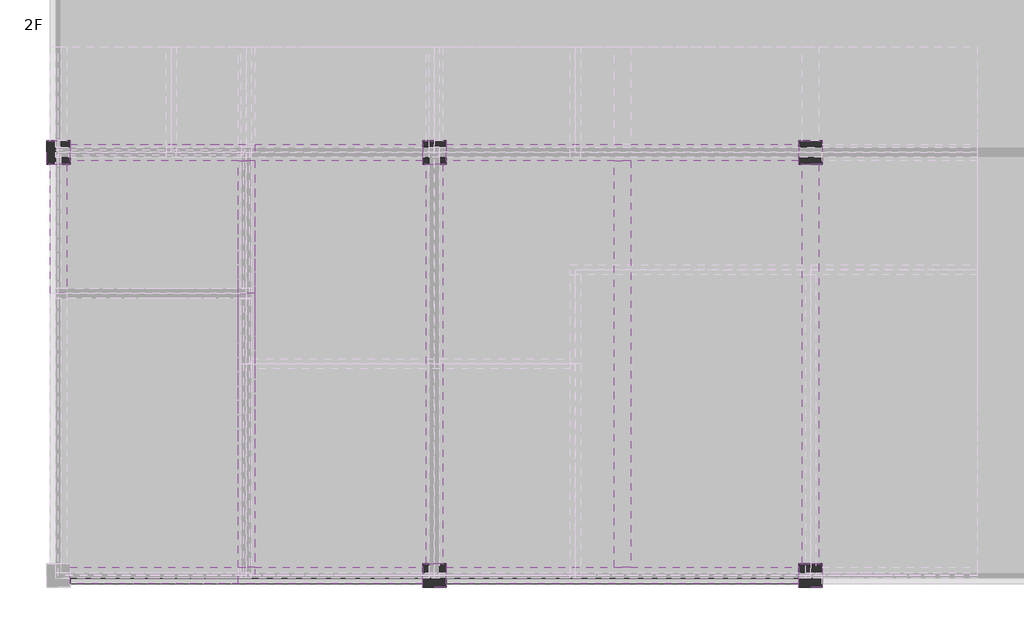
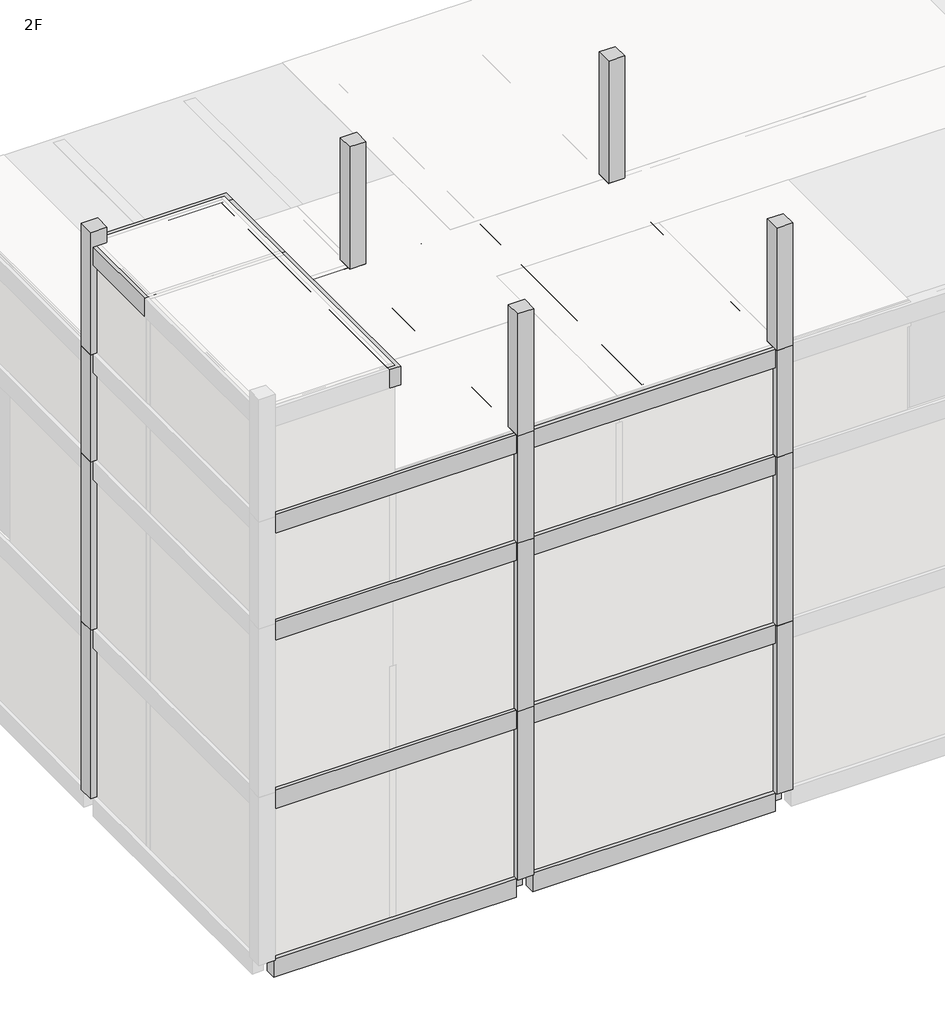
# One storey, part 4 of 7: 36 beams, 20 columns.
"""IFC4 building model written with IfcOpenShell, lengths in millimetres."""

from ifc_helpers import new_model, si_unit, frame, origin, place, context, project, spatial, polyline, outline, extrude, faceted_brep, element, save

model = new_model("IFC4")

# Units and contexts
model_context = context("Model", 3, world=origin())
ifc_project = project(units=[si_unit("LENGTHUNIT", "METRE", prefix="MILLI")], contexts=[model_context])

# Site, building, storey
site = spatial("IfcSite", under=ifc_project)
building = spatial("IfcBuilding", under=site)
storey = spatial("IfcBuildingStorey", under=building, Name="2F", Elevation=3500.0)

# Beams
placement = place(None, origin())
element("IfcBeam", 1, ObjectType="Concrete-Rectangular-Beam : BM111_400x500_RG1", at=placement, inside=storey, context=model_context, shape_type="Brep", body=[
    faceted_brep([(49634.6521483, 169923.8614395, 21500.0), (49284.6521483, 169923.8614395, 21500.0), (49284.6521483, 164098.8614395, 21500.0), (49284.6521483, 163748.8614395, 21500.0), (49634.6521483, 163748.8614395, 21500.0), (49634.6521483, 169923.8614395, 20900.0), (49634.6521483, 163748.8614395, 20900.0), (49284.6521483, 169923.8614395, 20900.0), (49284.6521483, 163748.8614395, 20900.0), (49284.6521483, 164098.8614395, 20900.0)], [[[0, 1, 2, 3, 4]], [[5, 0, 4, 6]], [[7, 5, 6, 8, 9]], [[1, 7, 9, 8, 3, 2]], [[4, 3, 8, 6]], [[1, 0, 5, 7]]]),
])
element("IfcBeam", 2, ObjectType="Concrete-Rectangular-Beam : BM111_400x500_RG1", at=placement, inside=storey, context=model_context, shape_type="Brep", body=[
    faceted_brep([(49634.6521483, 172748.8614395, 21500.0), (49634.6521483, 173098.8614395, 21500.0), (45709.6521483, 173098.8614395, 21500.0), (45709.6521483, 172748.8614395, 21500.0), (49284.6521483, 172748.8614395, 21500.0), (49634.6521483, 173098.8614395, 20900.0), (45709.6521483, 173098.8614395, 20900.0), (49634.6521483, 172748.8614395, 20900.0), (49284.6521483, 172748.8614395, 20900.0), (45709.6521483, 172748.8614395, 20900.0)], [[[0, 1, 2, 3, 4]], [[1, 5, 6, 2]], [[5, 7, 8, 9, 6]], [[7, 0, 4, 3, 9, 8]], [[1, 0, 7, 5]], [[3, 2, 6, 9]]]),
])
element("IfcBeam", 3, ObjectType="Concrete-Rectangular-Beam : BM111_400x500_RG1", at=placement, inside=storey, context=model_context, shape_type="SweptSolid", body=[
    extrude(outline(polyline([(49634.6521483, 169923.8614395), (49284.6521483, 169923.8614395), (49284.6521483, 172748.8614395), (49634.6521483, 172748.8614395), (49634.6521483, 169923.8614395)])), frame((0.0, 0.0, 20900.0), z_axis=(0.0, 0.0, 1.0), x_axis=(1.0, 0.0, 0.0)), (0.0, 0.0, 1.0), 600.0),
])
element("IfcBeam", 4, ObjectType="Concrete-Rectangular-Beam : BM111_400x500_RG1", at=placement, inside=storey, context=model_context, shape_type="SweptSolid", body=[
    extrude(outline(polyline([(45634.6521483, 169923.8614395), (45284.6521483, 169923.8614395), (45284.6521483, 172673.8614395), (45634.6521483, 172673.8614395), (45634.6521483, 169923.8614395)])), frame((0.0, 0.0, 20900.0), z_axis=(0.0, 0.0, 1.0), x_axis=(1.0, 0.0, 0.0)), (0.0, 0.0, 1.0), 600.0),
])
element("IfcBeam", 5, ObjectType="Concrete-Rectangular-Beam : BM111_400x500_RG1", at=placement, inside=storey, context=model_context, shape_type="SweptSolid", body=[
    extrude(outline(polyline([(49284.6521483, 172748.8614395), (49634.6521483, 172748.8614395), (49634.6521483, 164098.8614395), (49284.6521483, 164098.8614395), (49284.6521483, 172748.8614395)])), frame((0.0, 0.0, 2900.0), z_axis=(0.0, 0.0, 1.0), x_axis=(1.0, 0.0, 0.0)), (0.0, 0.0, 1.0), 600.0),
])
element("IfcBeam", 6, ObjectType="Concrete-Rectangular-Beam : BM111_400x500_RG1", at=placement, inside=storey, context=model_context, shape_type="SweptSolid", body=[
    extrude(outline(polyline([(57284.6521483, 172748.8614395), (57634.6521483, 172748.8614395), (57634.6521483, 164098.8614395), (57284.6521483, 164098.8614395), (57284.6521483, 172748.8614395)])), frame((0.0, 0.0, 2900.0), z_axis=(0.0, 0.0, 1.0), x_axis=(1.0, 0.0, 0.0)), (0.0, 0.0, 1.0), 600.0),
])
element("IfcBeam", 7, ObjectType="Concrete-Rectangular-Beam : BM111_400x500_RG1", at=placement, inside=storey, context=model_context, shape_type="SweptSolid", body=[
    extrude(outline(polyline([(49284.6521483, 172748.8614395), (49634.6521483, 172748.8614395), (49634.6521483, 164098.8614395), (49284.6521483, 164098.8614395), (49284.6521483, 172748.8614395)])), frame((0.0, 0.0, 8400.0), z_axis=(0.0, 0.0, 1.0), x_axis=(1.0, 0.0, 0.0)), (0.0, 0.0, 1.0), 600.0),
])
element("IfcBeam", 8, ObjectType="Concrete-Rectangular-Beam : BM111_400x500_RG1", at=placement, inside=storey, context=model_context, shape_type="SweptSolid", body=[
    extrude(outline(polyline([(57284.6521483, 172748.8614395), (57634.6521483, 172748.8614395), (57634.6521483, 164098.8614395), (57284.6521483, 164098.8614395), (57284.6521483, 172748.8614395)])), frame((0.0, 0.0, 8400.0), z_axis=(0.0, 0.0, 1.0), x_axis=(1.0, 0.0, 0.0)), (0.0, 0.0, 1.0), 600.0),
])
element("IfcBeam", 9, ObjectType="Concrete-Rectangular-Beam : BM111_400x500_RG1", at=placement, inside=storey, context=model_context, shape_type="SweptSolid", body=[
    extrude(outline(polyline([(49284.6521483, 172748.8614395), (49634.6521483, 172748.8614395), (49634.6521483, 164098.8614395), (49284.6521483, 164098.8614395), (49284.6521483, 172748.8614395)])), frame((0.0, 0.0, 13900.0), z_axis=(0.0, 0.0, 1.0), x_axis=(1.0, 0.0, 0.0)), (0.0, 0.0, 1.0), 600.0),
])
element("IfcBeam", 10, ObjectType="Concrete-Rectangular-Beam : BM111_400x500_RG1", at=placement, inside=storey, context=model_context, shape_type="SweptSolid", body=[
    extrude(outline(polyline([(57284.6521483, 172748.8614395), (57634.6521483, 172748.8614395), (57634.6521483, 164098.8614395), (57284.6521483, 164098.8614395), (57284.6521483, 172748.8614395)])), frame((0.0, 0.0, 13900.0), z_axis=(0.0, 0.0, 1.0), x_axis=(1.0, 0.0, 0.0)), (0.0, 0.0, 1.0), 600.0),
])
element("IfcBeam", 11, ObjectType="Concrete-Rectangular-Beam : BM111_400x500_RG1", at=placement, inside=storey, context=model_context, shape_type="SweptSolid", body=[
    extrude(outline(polyline([(49284.6521483, 172748.8614395), (49634.6521483, 172748.8614395), (49634.6521483, 164098.8614395), (49284.6521483, 164098.8614395), (49284.6521483, 172748.8614395)])), frame((0.0, 0.0, 17400.0), z_axis=(0.0, 0.0, 1.0), x_axis=(1.0, 0.0, 0.0)), (0.0, 0.0, 1.0), 600.0),
])
element("IfcBeam", 12, ObjectType="Concrete-Rectangular-Beam : BM111_400x500_RG1", at=placement, inside=storey, context=model_context, shape_type="SweptSolid", body=[
    extrude(outline(polyline([(57284.6521483, 172748.8614395), (57634.6521483, 172748.8614395), (57634.6521483, 164098.8614395), (57284.6521483, 164098.8614395), (57284.6521483, 172748.8614395)])), frame((0.0, 0.0, 17400.0), z_axis=(0.0, 0.0, 1.0), x_axis=(1.0, 0.0, 0.0)), (0.0, 0.0, 1.0), 600.0),
])
element("IfcBeam", 13, ObjectType="Concrete-Rectangular-Beam : BM111_400x500_RG1", at=placement, inside=storey, context=model_context, shape_type="Brep", body=[
    faceted_brep([(45709.6521483, 173098.8614395, 3500.0), (45709.6521483, 172748.8614395, 3500.0), (49284.6521483, 172748.8614395, 3500.0), (49634.6521483, 172748.8614395, 3500.0), (53209.6521483, 172748.8614395, 3500.0), (53209.6521483, 173098.8614395, 3500.0), (49634.6521483, 173098.8614395, 3500.0), (49284.6521483, 173098.8614395, 3500.0), (45709.6521483, 172748.8614395, 2900.0), (49284.6521483, 172748.8614395, 2900.0), (49634.6521483, 172748.8614395, 2900.0), (53209.6521483, 172748.8614395, 2900.0), (45709.6521483, 173098.8614395, 2900.0), (49284.6521483, 173098.8614395, 2900.0), (49634.6521483, 173098.8614395, 2900.0), (53209.6521483, 173098.8614395, 2900.0)], [[[0, 1, 2, 3, 4, 5, 6, 7]], [[1, 8, 9, 10, 11, 4, 3, 2]], [[8, 12, 13, 14, 15, 11, 10, 9]], [[12, 0, 7, 6, 5, 15, 14, 13]], [[1, 0, 12, 8]], [[5, 4, 11, 15]]]),
])
element("IfcBeam", 14, ObjectType="Concrete-Rectangular-Beam : BM111_400x500_RG1", at=placement, inside=storey, context=model_context, shape_type="Brep", body=[
    faceted_brep([(53709.6521483, 173098.8614395, 3500.0), (53709.6521483, 172748.8614395, 3500.0), (57284.6521483, 172748.8614395, 3500.0), (57634.6521483, 172748.8614395, 3500.0), (61209.6521483, 172748.8614395, 3500.0), (61209.6521483, 173098.8614395, 3500.0), (57634.6521483, 173098.8614395, 3500.0), (57284.6521483, 173098.8614395, 3500.0), (53709.6521483, 172748.8614395, 2900.0), (57284.6521483, 172748.8614395, 2900.0), (57634.6521483, 172748.8614395, 2900.0), (61209.6521483, 172748.8614395, 2900.0), (53709.6521483, 173098.8614395, 2900.0), (57284.6521483, 173098.8614395, 2900.0), (57634.6521483, 173098.8614395, 2900.0), (61209.6521483, 173098.8614395, 2900.0)], [[[0, 1, 2, 3, 4, 5, 6, 7]], [[1, 8, 9, 10, 11, 4, 3, 2]], [[8, 12, 13, 14, 15, 11, 10, 9]], [[12, 0, 7, 6, 5, 15, 14, 13]], [[1, 0, 12, 8]], [[5, 4, 11, 15]]]),
])
element("IfcBeam", 15, ObjectType="Concrete-Rectangular-Beam : BM111_400x500_RG1", at=placement, inside=storey, context=model_context, shape_type="Brep", body=[
    faceted_brep([(45709.6521483, 164098.8614395, 3500.0), (45709.6521483, 163748.8614395, 3500.0), (53209.6521483, 163748.8614395, 3500.0), (53209.6521483, 164098.8614395, 3500.0), (49634.6521483, 164098.8614395, 3500.0), (49284.6521483, 164098.8614395, 3500.0), (45709.6521483, 163748.8614395, 2900.0), (53209.6521483, 163748.8614395, 2900.0), (45709.6521483, 164098.8614395, 2900.0), (49284.6521483, 164098.8614395, 2900.0), (49634.6521483, 164098.8614395, 2900.0), (53209.6521483, 164098.8614395, 2900.0)], [[[0, 1, 2, 3, 4, 5]], [[1, 6, 7, 2]], [[6, 8, 9, 10, 11, 7]], [[8, 0, 5, 4, 3, 11, 10, 9]], [[1, 0, 8, 6]], [[3, 2, 7, 11]]]),
])
element("IfcBeam", 16, ObjectType="Concrete-Rectangular-Beam : BM111_400x500_RG1", at=placement, inside=storey, context=model_context, shape_type="Brep", body=[
    faceted_brep([(53709.6521483, 164098.8614395, 3500.0), (53709.6521483, 163748.8614395, 3500.0), (61209.6521483, 163748.8614395, 3500.0), (61209.6521483, 164098.8614395, 3500.0), (57634.6521483, 164098.8614395, 3500.0), (57284.6521483, 164098.8614395, 3500.0), (53709.6521483, 163748.8614395, 2900.0), (61209.6521483, 163748.8614395, 2900.0), (53709.6521483, 164098.8614395, 2900.0), (57284.6521483, 164098.8614395, 2900.0), (57634.6521483, 164098.8614395, 2900.0), (61209.6521483, 164098.8614395, 2900.0)], [[[0, 1, 2, 3, 4, 5]], [[1, 6, 7, 2]], [[6, 8, 9, 10, 11, 7]], [[8, 0, 5, 4, 3, 11, 10, 9]], [[1, 0, 8, 6]], [[3, 2, 7, 11]]]),
])
element("IfcBeam", 17, ObjectType="Concrete-Rectangular-Beam : BM111_400x500_RG1", at=placement, inside=storey, context=model_context, shape_type="Brep", body=[
    faceted_brep([(45709.6521483, 173098.8614395, 9000.0), (45709.6521483, 172748.8614395, 9000.0), (49284.6521483, 172748.8614395, 9000.0), (49634.6521483, 172748.8614395, 9000.0), (53209.6521483, 172748.8614395, 9000.0), (53209.6521483, 173098.8614395, 9000.0), (49634.6521483, 173098.8614395, 9000.0), (49284.6521483, 173098.8614395, 9000.0), (45709.6521483, 172748.8614395, 8400.0), (49284.6521483, 172748.8614395, 8400.0), (49634.6521483, 172748.8614395, 8400.0), (53209.6521483, 172748.8614395, 8400.0), (45709.6521483, 173098.8614395, 8400.0), (49284.6521483, 173098.8614395, 8400.0), (49634.6521483, 173098.8614395, 8400.0), (53209.6521483, 173098.8614395, 8400.0)], [[[0, 1, 2, 3, 4, 5, 6, 7]], [[1, 8, 9, 10, 11, 4, 3, 2]], [[8, 12, 13, 14, 15, 11, 10, 9]], [[12, 0, 7, 6, 5, 15, 14, 13]], [[1, 0, 12, 8]], [[5, 4, 11, 15]]]),
])
element("IfcBeam", 18, ObjectType="Concrete-Rectangular-Beam : BM111_400x500_RG1", at=placement, inside=storey, context=model_context, shape_type="Brep", body=[
    faceted_brep([(53709.6521483, 173098.8614395, 9000.0), (53709.6521483, 172748.8614395, 9000.0), (57284.6521483, 172748.8614395, 9000.0), (57634.6521483, 172748.8614395, 9000.0), (61209.6521483, 172748.8614395, 9000.0), (61209.6521483, 173098.8614395, 9000.0), (57634.6521483, 173098.8614395, 9000.0), (57284.6521483, 173098.8614395, 9000.0), (53709.6521483, 172748.8614395, 8400.0), (57284.6521483, 172748.8614395, 8400.0), (57634.6521483, 172748.8614395, 8400.0), (61209.6521483, 172748.8614395, 8400.0), (53709.6521483, 173098.8614395, 8400.0), (57284.6521483, 173098.8614395, 8400.0), (57634.6521483, 173098.8614395, 8400.0), (61209.6521483, 173098.8614395, 8400.0)], [[[0, 1, 2, 3, 4, 5, 6, 7]], [[1, 8, 9, 10, 11, 4, 3, 2]], [[8, 12, 13, 14, 15, 11, 10, 9]], [[12, 0, 7, 6, 5, 15, 14, 13]], [[1, 0, 12, 8]], [[5, 4, 11, 15]]]),
])
element("IfcBeam", 19, ObjectType="Concrete-Rectangular-Beam : BM111_400x500_RG1", at=placement, inside=storey, context=model_context, shape_type="Brep", body=[
    faceted_brep([(45709.6521483, 164098.8614395, 9000.0), (45709.6521483, 163748.8614395, 9000.0), (53209.6521483, 163748.8614395, 9000.0), (53209.6521483, 164098.8614395, 9000.0), (49634.6521483, 164098.8614395, 9000.0), (49284.6521483, 164098.8614395, 9000.0), (45709.6521483, 163748.8614395, 8400.0), (53209.6521483, 163748.8614395, 8400.0), (45709.6521483, 164098.8614395, 8400.0), (49284.6521483, 164098.8614395, 8400.0), (49634.6521483, 164098.8614395, 8400.0), (53209.6521483, 164098.8614395, 8400.0)], [[[0, 1, 2, 3, 4, 5]], [[1, 6, 7, 2]], [[6, 8, 9, 10, 11, 7]], [[8, 0, 5, 4, 3, 11, 10, 9]], [[1, 0, 8, 6]], [[3, 2, 7, 11]]]),
])
element("IfcBeam", 20, ObjectType="Concrete-Rectangular-Beam : BM111_400x500_RG1", at=placement, inside=storey, context=model_context, shape_type="Brep", body=[
    faceted_brep([(53709.6521483, 164098.8614395, 9000.0), (53709.6521483, 163748.8614395, 9000.0), (61209.6521483, 163748.8614395, 9000.0), (61209.6521483, 164098.8614395, 9000.0), (57634.6521483, 164098.8614395, 9000.0), (57284.6521483, 164098.8614395, 9000.0), (53709.6521483, 163748.8614395, 8400.0), (61209.6521483, 163748.8614395, 8400.0), (53709.6521483, 164098.8614395, 8400.0), (57284.6521483, 164098.8614395, 8400.0), (57634.6521483, 164098.8614395, 8400.0), (61209.6521483, 164098.8614395, 8400.0)], [[[0, 1, 2, 3, 4, 5]], [[1, 6, 7, 2]], [[6, 8, 9, 10, 11, 7]], [[8, 0, 5, 4, 3, 11, 10, 9]], [[1, 0, 8, 6]], [[3, 2, 7, 11]]]),
])
element("IfcBeam", 21, ObjectType="Concrete-Rectangular-Beam : BM111_400x500_RG1", at=placement, inside=storey, context=model_context, shape_type="Brep", body=[
    faceted_brep([(45709.6521483, 173098.8614395, 14500.0), (45709.6521483, 172748.8614395, 14500.0), (49284.6521483, 172748.8614395, 14500.0), (49634.6521483, 172748.8614395, 14500.0), (53209.6521483, 172748.8614395, 14500.0), (53209.6521483, 173098.8614395, 14500.0), (49634.6521483, 173098.8614395, 14500.0), (49284.6521483, 173098.8614395, 14500.0), (45709.6521483, 172748.8614395, 13900.0), (49284.6521483, 172748.8614395, 13900.0), (49634.6521483, 172748.8614395, 13900.0), (53209.6521483, 172748.8614395, 13900.0), (45709.6521483, 173098.8614395, 13900.0), (49284.6521483, 173098.8614395, 13900.0), (49634.6521483, 173098.8614395, 13900.0), (53209.6521483, 173098.8614395, 13900.0)], [[[0, 1, 2, 3, 4, 5, 6, 7]], [[1, 8, 9, 10, 11, 4, 3, 2]], [[8, 12, 13, 14, 15, 11, 10, 9]], [[12, 0, 7, 6, 5, 15, 14, 13]], [[1, 0, 12, 8]], [[5, 4, 11, 15]]]),
])
element("IfcBeam", 22, ObjectType="Concrete-Rectangular-Beam : BM111_400x500_RG1", at=placement, inside=storey, context=model_context, shape_type="Brep", body=[
    faceted_brep([(53709.6521483, 173098.8614395, 14500.0), (53709.6521483, 172748.8614395, 14500.0), (57284.6521483, 172748.8614395, 14500.0), (57634.6521483, 172748.8614395, 14500.0), (61209.6521483, 172748.8614395, 14500.0), (61209.6521483, 173098.8614395, 14500.0), (57634.6521483, 173098.8614395, 14500.0), (57284.6521483, 173098.8614395, 14500.0), (53709.6521483, 172748.8614395, 13900.0), (57284.6521483, 172748.8614395, 13900.0), (57634.6521483, 172748.8614395, 13900.0), (61209.6521483, 172748.8614395, 13900.0), (53709.6521483, 173098.8614395, 13900.0), (57284.6521483, 173098.8614395, 13900.0), (57634.6521483, 173098.8614395, 13900.0), (61209.6521483, 173098.8614395, 13900.0)], [[[0, 1, 2, 3, 4, 5, 6, 7]], [[1, 8, 9, 10, 11, 4, 3, 2]], [[8, 12, 13, 14, 15, 11, 10, 9]], [[12, 0, 7, 6, 5, 15, 14, 13]], [[1, 0, 12, 8]], [[5, 4, 11, 15]]]),
])
element("IfcBeam", 23, ObjectType="Concrete-Rectangular-Beam : BM111_400x500_RG1", at=placement, inside=storey, context=model_context, shape_type="Brep", body=[
    faceted_brep([(45709.6521483, 164098.8614395, 14500.0), (45709.6521483, 163748.8614395, 14500.0), (53209.6521483, 163748.8614395, 14500.0), (53209.6521483, 164098.8614395, 14500.0), (49634.6521483, 164098.8614395, 14500.0), (49284.6521483, 164098.8614395, 14500.0), (45709.6521483, 163748.8614395, 13900.0), (53209.6521483, 163748.8614395, 13900.0), (45709.6521483, 164098.8614395, 13900.0), (49284.6521483, 164098.8614395, 13900.0), (49634.6521483, 164098.8614395, 13900.0), (53209.6521483, 164098.8614395, 13900.0)], [[[0, 1, 2, 3, 4, 5]], [[1, 6, 7, 2]], [[6, 8, 9, 10, 11, 7]], [[8, 0, 5, 4, 3, 11, 10, 9]], [[1, 0, 8, 6]], [[3, 2, 7, 11]]]),
])
element("IfcBeam", 24, ObjectType="Concrete-Rectangular-Beam : BM111_400x500_RG1", at=placement, inside=storey, context=model_context, shape_type="Brep", body=[
    faceted_brep([(53709.6521483, 164098.8614395, 14500.0), (53709.6521483, 163748.8614395, 14500.0), (61209.6521483, 163748.8614395, 14500.0), (61209.6521483, 164098.8614395, 14500.0), (57634.6521483, 164098.8614395, 14500.0), (57284.6521483, 164098.8614395, 14500.0), (53709.6521483, 163748.8614395, 13900.0), (61209.6521483, 163748.8614395, 13900.0), (53709.6521483, 164098.8614395, 13900.0), (57284.6521483, 164098.8614395, 13900.0), (57634.6521483, 164098.8614395, 13900.0), (61209.6521483, 164098.8614395, 13900.0)], [[[0, 1, 2, 3, 4, 5]], [[1, 6, 7, 2]], [[6, 8, 9, 10, 11, 7]], [[8, 0, 5, 4, 3, 11, 10, 9]], [[1, 0, 8, 6]], [[3, 2, 7, 11]]]),
])
element("IfcBeam", 25, ObjectType="Concrete-Rectangular-Beam : BM111_400x500_RG1", at=placement, inside=storey, context=model_context, shape_type="Brep", body=[
    faceted_brep([(45709.6521483, 173098.8614395, 18000.0), (45709.6521483, 172748.8614395, 18000.0), (49284.6521483, 172748.8614395, 18000.0), (49634.6521483, 172748.8614395, 18000.0), (53209.6521483, 172748.8614395, 18000.0), (53209.6521483, 173098.8614395, 18000.0), (49634.6521483, 173098.8614395, 18000.0), (49284.6521483, 173098.8614395, 18000.0), (45709.6521483, 172748.8614395, 17400.0), (49284.6521483, 172748.8614395, 17400.0), (49634.6521483, 172748.8614395, 17400.0), (53209.6521483, 172748.8614395, 17400.0), (45709.6521483, 173098.8614395, 17400.0), (49284.6521483, 173098.8614395, 17400.0), (49634.6521483, 173098.8614395, 17400.0), (53209.6521483, 173098.8614395, 17400.0)], [[[0, 1, 2, 3, 4, 5, 6, 7]], [[1, 8, 9, 10, 11, 4, 3, 2]], [[8, 12, 13, 14, 15, 11, 10, 9]], [[12, 0, 7, 6, 5, 15, 14, 13]], [[1, 0, 12, 8]], [[5, 4, 11, 15]]]),
])
element("IfcBeam", 26, ObjectType="Concrete-Rectangular-Beam : BM111_400x500_RG1", at=placement, inside=storey, context=model_context, shape_type="Brep", body=[
    faceted_brep([(53709.6521483, 173098.8614395, 18000.0), (53709.6521483, 172748.8614395, 18000.0), (57284.6521483, 172748.8614395, 18000.0), (57634.6521483, 172748.8614395, 18000.0), (61209.6521483, 172748.8614395, 18000.0), (61209.6521483, 173098.8614395, 18000.0), (57634.6521483, 173098.8614395, 18000.0), (57284.6521483, 173098.8614395, 18000.0), (53709.6521483, 172748.8614395, 17400.0), (57284.6521483, 172748.8614395, 17400.0), (57634.6521483, 172748.8614395, 17400.0), (61209.6521483, 172748.8614395, 17400.0), (53709.6521483, 173098.8614395, 17400.0), (57284.6521483, 173098.8614395, 17400.0), (57634.6521483, 173098.8614395, 17400.0), (61209.6521483, 173098.8614395, 17400.0)], [[[0, 1, 2, 3, 4, 5, 6, 7]], [[1, 8, 9, 10, 11, 4, 3, 2]], [[8, 12, 13, 14, 15, 11, 10, 9]], [[12, 0, 7, 6, 5, 15, 14, 13]], [[1, 0, 12, 8]], [[5, 4, 11, 15]]]),
])
element("IfcBeam", 27, ObjectType="Concrete-Rectangular-Beam : BM111_400x500_RG1", at=placement, inside=storey, context=model_context, shape_type="Brep", body=[
    faceted_brep([(45709.6521483, 164098.8614395, 18000.0), (45709.6521483, 163748.8614395, 18000.0), (53209.6521483, 163748.8614395, 18000.0), (53209.6521483, 164098.8614395, 18000.0), (49634.6521483, 164098.8614395, 18000.0), (49284.6521483, 164098.8614395, 18000.0), (45709.6521483, 163748.8614395, 17400.0), (53209.6521483, 163748.8614395, 17400.0), (45709.6521483, 164098.8614395, 17400.0), (49284.6521483, 164098.8614395, 17400.0), (49634.6521483, 164098.8614395, 17400.0), (53209.6521483, 164098.8614395, 17400.0)], [[[0, 1, 2, 3, 4, 5]], [[1, 6, 7, 2]], [[6, 8, 9, 10, 11, 7]], [[8, 0, 5, 4, 3, 11, 10, 9]], [[1, 0, 8, 6]], [[3, 2, 7, 11]]]),
])
element("IfcBeam", 28, ObjectType="Concrete-Rectangular-Beam : BM111_400x500_RG1", at=placement, inside=storey, context=model_context, shape_type="Brep", body=[
    faceted_brep([(53709.6521483, 164098.8614395, 18000.0), (53709.6521483, 163748.8614395, 18000.0), (61209.6521483, 163748.8614395, 18000.0), (61209.6521483, 164098.8614395, 18000.0), (57634.6521483, 164098.8614395, 18000.0), (57284.6521483, 164098.8614395, 18000.0), (53709.6521483, 163748.8614395, 17400.0), (61209.6521483, 163748.8614395, 17400.0), (53709.6521483, 164098.8614395, 17400.0), (57284.6521483, 164098.8614395, 17400.0), (57634.6521483, 164098.8614395, 17400.0), (61209.6521483, 164098.8614395, 17400.0)], [[[0, 1, 2, 3, 4, 5]], [[1, 6, 7, 2]], [[6, 8, 9, 10, 11, 7]], [[8, 0, 5, 4, 3, 11, 10, 9]], [[1, 0, 8, 6]], [[3, 2, 7, 11]]]),
])
element("IfcBeam", 29, ObjectType="Concrete-Rectangular-Beam : BM111_400x500_RG1", at=placement, inside=storey, context=model_context, shape_type="SweptSolid", body=[
    extrude(outline(polyline([(53284.6521483, 172673.8614395), (53634.6521483, 172673.8614395), (53634.6521483, 164173.8614395), (53284.6521483, 164173.8614395), (53284.6521483, 172673.8614395)])), frame((0.0, 0.0, 2900.0), z_axis=(0.0, 0.0, 1.0), x_axis=(1.0, 0.0, 0.0)), (0.0, 0.0, 1.0), 600.0),
])
element("IfcBeam", 30, ObjectType="Concrete-Rectangular-Beam : BM111_400x500_RG1", at=placement, inside=storey, context=model_context, shape_type="SweptSolid", body=[
    extrude(outline(polyline([(61284.6521483, 172673.8614395), (61634.6521483, 172673.8614395), (61634.6521483, 164173.8614395), (61284.6521483, 164173.8614395), (61284.6521483, 172673.8614395)])), frame((0.0, 0.0, 2900.0), z_axis=(0.0, 0.0, 1.0), x_axis=(1.0, 0.0, 0.0)), (0.0, 0.0, 1.0), 600.0),
])
element("IfcBeam", 31, ObjectType="Concrete-Rectangular-Beam : BM111_400x500_RG1", at=placement, inside=storey, context=model_context, shape_type="SweptSolid", body=[
    extrude(outline(polyline([(53284.6521483, 172673.8614395), (53634.6521483, 172673.8614395), (53634.6521483, 164173.8614395), (53284.6521483, 164173.8614395), (53284.6521483, 172673.8614395)])), frame((0.0, 0.0, 8400.0), z_axis=(0.0, 0.0, 1.0), x_axis=(1.0, 0.0, 0.0)), (0.0, 0.0, 1.0), 600.0),
])
element("IfcBeam", 32, ObjectType="Concrete-Rectangular-Beam : BM111_400x500_RG1", at=placement, inside=storey, context=model_context, shape_type="SweptSolid", body=[
    extrude(outline(polyline([(61284.6521483, 172673.8614395), (61634.6521483, 172673.8614395), (61634.6521483, 164173.8614395), (61284.6521483, 164173.8614395), (61284.6521483, 172673.8614395)])), frame((0.0, 0.0, 8400.0), z_axis=(0.0, 0.0, 1.0), x_axis=(1.0, 0.0, 0.0)), (0.0, 0.0, 1.0), 600.0),
])
element("IfcBeam", 33, ObjectType="Concrete-Rectangular-Beam : BM111_400x500_RG1", at=placement, inside=storey, context=model_context, shape_type="SweptSolid", body=[
    extrude(outline(polyline([(53284.6521483, 172673.8614395), (53634.6521483, 172673.8614395), (53634.6521483, 164173.8614395), (53284.6521483, 164173.8614395), (53284.6521483, 172673.8614395)])), frame((0.0, 0.0, 13900.0), z_axis=(0.0, 0.0, 1.0), x_axis=(1.0, 0.0, 0.0)), (0.0, 0.0, 1.0), 600.0),
])
element("IfcBeam", 34, ObjectType="Concrete-Rectangular-Beam : BM111_400x500_RG1", at=placement, inside=storey, context=model_context, shape_type="SweptSolid", body=[
    extrude(outline(polyline([(61284.6521483, 172673.8614395), (61634.6521483, 172673.8614395), (61634.6521483, 164173.8614395), (61284.6521483, 164173.8614395), (61284.6521483, 172673.8614395)])), frame((0.0, 0.0, 13900.0), z_axis=(0.0, 0.0, 1.0), x_axis=(1.0, 0.0, 0.0)), (0.0, 0.0, 1.0), 600.0),
])
element("IfcBeam", 35, ObjectType="Concrete-Rectangular-Beam : BM111_400x500_RG1", at=placement, inside=storey, context=model_context, shape_type="SweptSolid", body=[
    extrude(outline(polyline([(53284.6521483, 172673.8614395), (53634.6521483, 172673.8614395), (53634.6521483, 164173.8614395), (53284.6521483, 164173.8614395), (53284.6521483, 172673.8614395)])), frame((0.0, 0.0, 17400.0), z_axis=(0.0, 0.0, 1.0), x_axis=(1.0, 0.0, 0.0)), (0.0, 0.0, 1.0), 600.0),
])
element("IfcBeam", 36, ObjectType="Concrete-Rectangular-Beam : BM111_400x500_RG1", at=placement, inside=storey, context=model_context, shape_type="SweptSolid", body=[
    extrude(outline(polyline([(61284.6521483, 172673.8614395), (61634.6521483, 172673.8614395), (61634.6521483, 164173.8614395), (61284.6521483, 164173.8614395), (61284.6521483, 172673.8614395)])), frame((0.0, 0.0, 17400.0), z_axis=(0.0, 0.0, 1.0), x_axis=(1.0, 0.0, 0.0)), (0.0, 0.0, 1.0), 600.0),
])

# Columns
element("IfcColumn", 37, ObjectType="Concrete-Rectangular-Column : CL111_500x500", at=placement, inside=storey, context=model_context, shape_type="Brep", body=[
    faceted_brep([(45709.6521483, 173173.8614395, 3500.0), (45709.6521483, 172673.8614395, 3500.0), (45209.6521483, 172673.8614395, 3500.0), (45209.6521483, 173173.8614395, 3500.0), (45709.6521483, 173173.8614395, 9000.0), (45709.6521483, 173098.8614395, 9000.0), (45709.6521483, 172748.8614395, 9000.0), (45709.6521483, 172673.8614395, 9000.0), (45634.6521483, 172673.8614395, 9000.0), (45284.6521483, 172673.8614395, 9000.0), (45209.6521483, 172673.8614395, 9000.0), (45209.6521483, 173173.8614395, 9000.0), (45284.6521483, 173173.8614395, 9000.0), (45634.6521483, 173173.8614395, 9000.0)], [[[0, 1, 2, 3]], [[4, 5, 6, 7, 1, 0]], [[7, 8, 9, 10, 2, 1]], [[10, 11, 3, 2]], [[11, 12, 13, 4, 0, 3]], [[4, 13, 12, 11, 10, 9, 8, 7, 6, 5]]]),
])
element("IfcColumn", 38, ObjectType="Concrete-Rectangular-Column : CL111_500x500", at=placement, inside=storey, context=model_context, shape_type="Brep", body=[
    faceted_brep([(45709.6521483, 173173.8614395, 9000.0), (45709.6521483, 172673.8614395, 9000.0), (45209.6521483, 172673.8614395, 9000.0), (45209.6521483, 173173.8614395, 9000.0), (45709.6521483, 173173.8614395, 14500.0), (45709.6521483, 173098.8614395, 14500.0), (45709.6521483, 172748.8614395, 14500.0), (45709.6521483, 172673.8614395, 14500.0), (45634.6521483, 172673.8614395, 14500.0), (45284.6521483, 172673.8614395, 14500.0), (45209.6521483, 172673.8614395, 14500.0), (45209.6521483, 173173.8614395, 14500.0), (45284.6521483, 173173.8614395, 14500.0), (45634.6521483, 173173.8614395, 14500.0)], [[[0, 1, 2, 3]], [[4, 5, 6, 7, 1, 0]], [[7, 8, 9, 10, 2, 1]], [[10, 11, 3, 2]], [[11, 12, 13, 4, 0, 3]], [[4, 13, 12, 11, 10, 9, 8, 7, 6, 5]]]),
])
element("IfcColumn", 39, ObjectType="Concrete-Rectangular-Column : CL111_500x500", at=placement, inside=storey, context=model_context, shape_type="Brep", body=[
    faceted_brep([(45709.6521483, 173173.8614395, 14500.0), (45709.6521483, 172673.8614395, 14500.0), (45209.6521483, 172673.8614395, 14500.0), (45209.6521483, 173173.8614395, 14500.0), (45709.6521483, 173173.8614395, 18000.0), (45709.6521483, 173098.8614395, 18000.0), (45709.6521483, 172748.8614395, 18000.0), (45709.6521483, 172673.8614395, 18000.0), (45634.6521483, 172673.8614395, 18000.0), (45284.6521483, 172673.8614395, 18000.0), (45209.6521483, 172673.8614395, 18000.0), (45209.6521483, 173173.8614395, 18000.0), (45284.6521483, 173173.8614395, 18000.0), (45634.6521483, 173173.8614395, 18000.0)], [[[0, 1, 2, 3]], [[4, 5, 6, 7, 1, 0]], [[7, 8, 9, 10, 2, 1]], [[10, 11, 3, 2]], [[11, 12, 13, 4, 0, 3]], [[4, 13, 12, 11, 10, 9, 8, 7, 6, 5]]]),
])
element("IfcColumn", 40, ObjectType="Concrete-Rectangular-Column : CL111_500x500", at=placement, inside=storey, context=model_context, shape_type="SweptSolid", body=[
    extrude(outline(polyline([(45709.6521483, 173173.8614395), (45709.6521483, 172673.8614395), (45209.6521483, 172673.8614395), (45209.6521483, 173173.8614395), (45709.6521483, 173173.8614395)])), frame((0.0, 0.0, 18000.0), z_axis=(0.0, 0.0, 1.0), x_axis=(1.0, 0.0, 0.0)), (0.0, 0.0, 1.0), 4000.0),
])
element("IfcColumn", 41, ObjectType="Concrete-Rectangular-Column : CL111_500x500", at=placement, inside=storey, context=model_context, shape_type="Brep", body=[
    faceted_brep([(53709.6521483, 173173.8614395, 3500.0), (53709.6521483, 172673.8614395, 3500.0), (53209.6521483, 172673.8614395, 3500.0), (53209.6521483, 173173.8614395, 3500.0), (53709.6521483, 173173.8614395, 9000.0), (53709.6521483, 173098.8614395, 9000.0), (53709.6521483, 172748.8614395, 9000.0), (53709.6521483, 172673.8614395, 9000.0), (53634.6521483, 172673.8614395, 9000.0), (53284.6521483, 172673.8614395, 9000.0), (53209.6521483, 172673.8614395, 9000.0), (53209.6521483, 172748.8614395, 9000.0), (53209.6521483, 173098.8614395, 9000.0), (53209.6521483, 173173.8614395, 9000.0), (53284.6521483, 173173.8614395, 9000.0), (53634.6521483, 173173.8614395, 9000.0)], [[[0, 1, 2, 3]], [[4, 5, 6, 7, 1, 0]], [[7, 8, 9, 10, 2, 1]], [[10, 11, 12, 13, 3, 2]], [[13, 14, 15, 4, 0, 3]], [[4, 15, 14, 13, 12, 11, 10, 9, 8, 7, 6, 5]]]),
])
element("IfcColumn", 42, ObjectType="Concrete-Rectangular-Column : CL111_500x500", at=placement, inside=storey, context=model_context, shape_type="Brep", body=[
    faceted_brep([(53709.6521483, 173173.8614395, 9000.0), (53709.6521483, 172673.8614395, 9000.0), (53209.6521483, 172673.8614395, 9000.0), (53209.6521483, 173173.8614395, 9000.0), (53709.6521483, 173173.8614395, 14500.0), (53709.6521483, 173098.8614395, 14500.0), (53709.6521483, 172748.8614395, 14500.0), (53709.6521483, 172673.8614395, 14500.0), (53634.6521483, 172673.8614395, 14500.0), (53284.6521483, 172673.8614395, 14500.0), (53209.6521483, 172673.8614395, 14500.0), (53209.6521483, 172748.8614395, 14500.0), (53209.6521483, 173098.8614395, 14500.0), (53209.6521483, 173173.8614395, 14500.0), (53284.6521483, 173173.8614395, 14500.0), (53634.6521483, 173173.8614395, 14500.0)], [[[0, 1, 2, 3]], [[4, 5, 6, 7, 1, 0]], [[7, 8, 9, 10, 2, 1]], [[10, 11, 12, 13, 3, 2]], [[13, 14, 15, 4, 0, 3]], [[4, 15, 14, 13, 12, 11, 10, 9, 8, 7, 6, 5]]]),
])
element("IfcColumn", 43, ObjectType="Concrete-Rectangular-Column : CL111_500x500", at=placement, inside=storey, context=model_context, shape_type="Brep", body=[
    faceted_brep([(53709.6521483, 173173.8614395, 14500.0), (53709.6521483, 172673.8614395, 14500.0), (53209.6521483, 172673.8614395, 14500.0), (53209.6521483, 173173.8614395, 14500.0), (53709.6521483, 173173.8614395, 18000.0), (53709.6521483, 173098.8614395, 18000.0), (53709.6521483, 172748.8614395, 18000.0), (53709.6521483, 172673.8614395, 18000.0), (53634.6521483, 172673.8614395, 18000.0), (53284.6521483, 172673.8614395, 18000.0), (53209.6521483, 172673.8614395, 18000.0), (53209.6521483, 172748.8614395, 18000.0), (53209.6521483, 173098.8614395, 18000.0), (53209.6521483, 173173.8614395, 18000.0), (53284.6521483, 173173.8614395, 18000.0), (53634.6521483, 173173.8614395, 18000.0)], [[[0, 1, 2, 3]], [[4, 5, 6, 7, 1, 0]], [[7, 8, 9, 10, 2, 1]], [[10, 11, 12, 13, 3, 2]], [[13, 14, 15, 4, 0, 3]], [[4, 15, 14, 13, 12, 11, 10, 9, 8, 7, 6, 5]]]),
])
element("IfcColumn", 44, ObjectType="Concrete-Rectangular-Column : CL111_500x500", at=placement, inside=storey, context=model_context, shape_type="SweptSolid", body=[
    extrude(outline(polyline([(53709.6521483, 173173.8614395), (53709.6521483, 172673.8614395), (53209.6521483, 172673.8614395), (53209.6521483, 173173.8614395), (53709.6521483, 173173.8614395)])), frame((0.0, 0.0, 18000.0), z_axis=(0.0, 0.0, 1.0), x_axis=(1.0, 0.0, 0.0)), (0.0, 0.0, 1.0), 4000.0),
])
element("IfcColumn", 45, ObjectType="Concrete-Rectangular-Column : CL111_500x500", at=placement, inside=storey, context=model_context, shape_type="Brep", body=[
    faceted_brep([(61709.6521483, 173173.8614395, 3500.0), (61709.6521483, 172673.8614395, 3500.0), (61209.6521483, 172673.8614395, 3500.0), (61209.6521483, 173173.8614395, 3500.0), (61709.6521483, 173173.8614395, 9000.0), (61709.6521483, 173098.8614395, 9000.0), (61709.6521483, 172748.8614395, 9000.0), (61709.6521483, 172673.8614395, 9000.0), (61634.6521483, 172673.8614395, 9000.0), (61284.6521483, 172673.8614395, 9000.0), (61209.6521483, 172673.8614395, 9000.0), (61209.6521483, 172748.8614395, 9000.0), (61209.6521483, 173098.8614395, 9000.0), (61209.6521483, 173173.8614395, 9000.0), (61284.6521483, 173173.8614395, 9000.0), (61634.6521483, 173173.8614395, 9000.0)], [[[0, 1, 2, 3]], [[4, 5, 6, 7, 1, 0]], [[7, 8, 9, 10, 2, 1]], [[10, 11, 12, 13, 3, 2]], [[13, 14, 15, 4, 0, 3]], [[4, 15, 14, 13, 12, 11, 10, 9, 8, 7, 6, 5]]]),
])
element("IfcColumn", 46, ObjectType="Concrete-Rectangular-Column : CL111_500x500", at=placement, inside=storey, context=model_context, shape_type="Brep", body=[
    faceted_brep([(61709.6521483, 173173.8614395, 9000.0), (61709.6521483, 172673.8614395, 9000.0), (61209.6521483, 172673.8614395, 9000.0), (61209.6521483, 173173.8614395, 9000.0), (61709.6521483, 173173.8614395, 14500.0), (61709.6521483, 173098.8614395, 14500.0), (61709.6521483, 172748.8614395, 14500.0), (61709.6521483, 172673.8614395, 14500.0), (61634.6521483, 172673.8614395, 14500.0), (61284.6521483, 172673.8614395, 14500.0), (61209.6521483, 172673.8614395, 14500.0), (61209.6521483, 172748.8614395, 14500.0), (61209.6521483, 173098.8614395, 14500.0), (61209.6521483, 173173.8614395, 14500.0), (61284.6521483, 173173.8614395, 14500.0), (61634.6521483, 173173.8614395, 14500.0)], [[[0, 1, 2, 3]], [[4, 5, 6, 7, 1, 0]], [[7, 8, 9, 10, 2, 1]], [[10, 11, 12, 13, 3, 2]], [[13, 14, 15, 4, 0, 3]], [[4, 15, 14, 13, 12, 11, 10, 9, 8, 7, 6, 5]]]),
])
element("IfcColumn", 47, ObjectType="Concrete-Rectangular-Column : CL111_500x500", at=placement, inside=storey, context=model_context, shape_type="Brep", body=[
    faceted_brep([(61709.6521483, 173173.8614395, 14500.0), (61709.6521483, 172673.8614395, 14500.0), (61209.6521483, 172673.8614395, 14500.0), (61209.6521483, 173173.8614395, 14500.0), (61709.6521483, 173173.8614395, 18000.0), (61709.6521483, 173098.8614395, 18000.0), (61709.6521483, 172748.8614395, 18000.0), (61709.6521483, 172673.8614395, 18000.0), (61634.6521483, 172673.8614395, 18000.0), (61284.6521483, 172673.8614395, 18000.0), (61209.6521483, 172673.8614395, 18000.0), (61209.6521483, 172748.8614395, 18000.0), (61209.6521483, 173098.8614395, 18000.0), (61209.6521483, 173173.8614395, 18000.0), (61284.6521483, 173173.8614395, 18000.0), (61634.6521483, 173173.8614395, 18000.0)], [[[0, 1, 2, 3]], [[4, 5, 6, 7, 1, 0]], [[7, 8, 9, 10, 2, 1]], [[10, 11, 12, 13, 3, 2]], [[13, 14, 15, 4, 0, 3]], [[4, 15, 14, 13, 12, 11, 10, 9, 8, 7, 6, 5]]]),
])
element("IfcColumn", 48, ObjectType="Concrete-Rectangular-Column : CL111_500x500", at=placement, inside=storey, context=model_context, shape_type="SweptSolid", body=[
    extrude(outline(polyline([(61709.6521483, 173173.8614395), (61709.6521483, 172673.8614395), (61209.6521483, 172673.8614395), (61209.6521483, 173173.8614395), (61709.6521483, 173173.8614395)])), frame((0.0, 0.0, 18000.0), z_axis=(0.0, 0.0, 1.0), x_axis=(1.0, 0.0, 0.0)), (0.0, 0.0, 1.0), 4000.0),
])
element("IfcColumn", 49, ObjectType="Concrete-Rectangular-Column : CL111_500x500", at=placement, inside=storey, context=model_context, shape_type="Brep", body=[
    faceted_brep([(53709.6521483, 164173.8614395, 3500.0), (53709.6521483, 163673.8614395, 3500.0), (53209.6521483, 163673.8614395, 3500.0), (53209.6521483, 164173.8614395, 3500.0), (53709.6521483, 164173.8614395, 9000.0), (53709.6521483, 164098.8614395, 9000.0), (53709.6521483, 163748.8614395, 9000.0), (53709.6521483, 163673.8614395, 9000.0), (53209.6521483, 163673.8614395, 9000.0), (53209.6521483, 163748.8614395, 9000.0), (53209.6521483, 164098.8614395, 9000.0), (53209.6521483, 164173.8614395, 9000.0), (53284.6521483, 164173.8614395, 9000.0), (53634.6521483, 164173.8614395, 9000.0)], [[[0, 1, 2, 3]], [[4, 5, 6, 7, 1, 0]], [[7, 8, 2, 1]], [[8, 9, 10, 11, 3, 2]], [[11, 12, 13, 4, 0, 3]], [[4, 13, 12, 11, 10, 9, 8, 7, 6, 5]]]),
])
element("IfcColumn", 50, ObjectType="Concrete-Rectangular-Column : CL111_500x500", at=placement, inside=storey, context=model_context, shape_type="Brep", body=[
    faceted_brep([(53709.6521483, 164173.8614395, 9000.0), (53709.6521483, 163673.8614395, 9000.0), (53209.6521483, 163673.8614395, 9000.0), (53209.6521483, 164173.8614395, 9000.0), (53709.6521483, 164173.8614395, 14500.0), (53709.6521483, 164098.8614395, 14500.0), (53709.6521483, 163748.8614395, 14500.0), (53709.6521483, 163673.8614395, 14500.0), (53209.6521483, 163673.8614395, 14500.0), (53209.6521483, 163748.8614395, 14500.0), (53209.6521483, 164098.8614395, 14500.0), (53209.6521483, 164173.8614395, 14500.0), (53284.6521483, 164173.8614395, 14500.0), (53634.6521483, 164173.8614395, 14500.0)], [[[0, 1, 2, 3]], [[4, 5, 6, 7, 1, 0]], [[7, 8, 2, 1]], [[8, 9, 10, 11, 3, 2]], [[11, 12, 13, 4, 0, 3]], [[4, 13, 12, 11, 10, 9, 8, 7, 6, 5]]]),
])
element("IfcColumn", 51, ObjectType="Concrete-Rectangular-Column : CL111_500x500", at=placement, inside=storey, context=model_context, shape_type="Brep", body=[
    faceted_brep([(53709.6521483, 164173.8614395, 14500.0), (53709.6521483, 163673.8614395, 14500.0), (53209.6521483, 163673.8614395, 14500.0), (53209.6521483, 164173.8614395, 14500.0), (53709.6521483, 164173.8614395, 18000.0), (53709.6521483, 164098.8614395, 18000.0), (53709.6521483, 163748.8614395, 18000.0), (53709.6521483, 163673.8614395, 18000.0), (53209.6521483, 163673.8614395, 18000.0), (53209.6521483, 163748.8614395, 18000.0), (53209.6521483, 164098.8614395, 18000.0), (53209.6521483, 164173.8614395, 18000.0), (53284.6521483, 164173.8614395, 18000.0), (53634.6521483, 164173.8614395, 18000.0)], [[[0, 1, 2, 3]], [[4, 5, 6, 7, 1, 0]], [[7, 8, 2, 1]], [[8, 9, 10, 11, 3, 2]], [[11, 12, 13, 4, 0, 3]], [[4, 13, 12, 11, 10, 9, 8, 7, 6, 5]]]),
])
element("IfcColumn", 52, ObjectType="Concrete-Rectangular-Column : CL111_500x500", at=placement, inside=storey, context=model_context, shape_type="SweptSolid", body=[
    extrude(outline(polyline([(53709.6521483, 164173.8614395), (53709.6521483, 163673.8614395), (53209.6521483, 163673.8614395), (53209.6521483, 164173.8614395), (53709.6521483, 164173.8614395)])), frame((0.0, 0.0, 18000.0), z_axis=(0.0, 0.0, 1.0), x_axis=(1.0, 0.0, 0.0)), (0.0, 0.0, 1.0), 4000.0),
])
element("IfcColumn", 53, ObjectType="Concrete-Rectangular-Column : CL111_500x500", at=placement, inside=storey, context=model_context, shape_type="Brep", body=[
    faceted_brep([(61709.6521483, 164173.8614395, 3500.0), (61709.6521483, 163673.8614395, 3500.0), (61209.6521483, 163673.8614395, 3500.0), (61209.6521483, 164173.8614395, 3500.0), (61709.6521483, 164173.8614395, 9000.0), (61709.6521483, 164098.8614395, 9000.0), (61709.6521483, 163748.8614395, 9000.0), (61709.6521483, 163673.8614395, 9000.0), (61209.6521483, 163673.8614395, 9000.0), (61209.6521483, 163748.8614395, 9000.0), (61209.6521483, 164098.8614395, 9000.0), (61209.6521483, 164173.8614395, 9000.0), (61284.6521483, 164173.8614395, 9000.0), (61634.6521483, 164173.8614395, 9000.0)], [[[0, 1, 2, 3]], [[4, 5, 6, 7, 1, 0]], [[7, 8, 2, 1]], [[8, 9, 10, 11, 3, 2]], [[11, 12, 13, 4, 0, 3]], [[4, 13, 12, 11, 10, 9, 8, 7, 6, 5]]]),
])
element("IfcColumn", 54, ObjectType="Concrete-Rectangular-Column : CL111_500x500", at=placement, inside=storey, context=model_context, shape_type="Brep", body=[
    faceted_brep([(61709.6521483, 164173.8614395, 9000.0), (61709.6521483, 163673.8614395, 9000.0), (61209.6521483, 163673.8614395, 9000.0), (61209.6521483, 164173.8614395, 9000.0), (61709.6521483, 164173.8614395, 14500.0), (61709.6521483, 164098.8614395, 14500.0), (61709.6521483, 163748.8614395, 14500.0), (61709.6521483, 163673.8614395, 14500.0), (61209.6521483, 163673.8614395, 14500.0), (61209.6521483, 163748.8614395, 14500.0), (61209.6521483, 164098.8614395, 14500.0), (61209.6521483, 164173.8614395, 14500.0), (61284.6521483, 164173.8614395, 14500.0), (61634.6521483, 164173.8614395, 14500.0)], [[[0, 1, 2, 3]], [[4, 5, 6, 7, 1, 0]], [[7, 8, 2, 1]], [[8, 9, 10, 11, 3, 2]], [[11, 12, 13, 4, 0, 3]], [[4, 13, 12, 11, 10, 9, 8, 7, 6, 5]]]),
])
element("IfcColumn", 55, ObjectType="Concrete-Rectangular-Column : CL111_500x500", at=placement, inside=storey, context=model_context, shape_type="Brep", body=[
    faceted_brep([(61709.6521483, 164173.8614395, 14500.0), (61709.6521483, 163673.8614395, 14500.0), (61209.6521483, 163673.8614395, 14500.0), (61209.6521483, 164173.8614395, 14500.0), (61709.6521483, 164173.8614395, 18000.0), (61709.6521483, 164098.8614395, 18000.0), (61709.6521483, 163748.8614395, 18000.0), (61709.6521483, 163673.8614395, 18000.0), (61209.6521483, 163673.8614395, 18000.0), (61209.6521483, 163748.8614395, 18000.0), (61209.6521483, 164098.8614395, 18000.0), (61209.6521483, 164173.8614395, 18000.0), (61284.6521483, 164173.8614395, 18000.0), (61634.6521483, 164173.8614395, 18000.0)], [[[0, 1, 2, 3]], [[4, 5, 6, 7, 1, 0]], [[7, 8, 2, 1]], [[8, 9, 10, 11, 3, 2]], [[11, 12, 13, 4, 0, 3]], [[4, 13, 12, 11, 10, 9, 8, 7, 6, 5]]]),
])
element("IfcColumn", 56, ObjectType="Concrete-Rectangular-Column : CL111_500x500", at=placement, inside=storey, context=model_context, shape_type="SweptSolid", body=[
    extrude(outline(polyline([(61709.6521483, 164173.8614395), (61709.6521483, 163673.8614395), (61209.6521483, 163673.8614395), (61209.6521483, 164173.8614395), (61709.6521483, 164173.8614395)])), frame((0.0, 0.0, 18000.0), z_axis=(0.0, 0.0, 1.0), x_axis=(1.0, 0.0, 0.0)), (0.0, 0.0, 1.0), 4000.0),
])

save(model, "model.ifc")

# Revit data of these elements
# Type "Concrete-Rectangular-Beam : BM111_400x500_RG1"
#   중앙부 하부근 = "3-D20"
#   중앙부 상부근 = "3-D20"
#   중앙부 보조근 = ""
#   중앙부 늑근 = "2-D10 @200"
#   외단부 하부근 = "3-D20"
#   외단부 상부근 = "3-D20"
#   외단부 보조근 = ""
#   외단부 늑근 = "2-D10 @100"
#   부호 = "RG1"
#   내단부 하부근 = "3-D20"
#   내단부 상부근 = "3-D20"
#   내단부 보조근 = ""
#   내단부 늑근 = "2-D10 @100"
#   ALL 하부근 = ""
#   ALL 상부근 = ""
#   ALL 보조근 = ""
#   ALL 늑근 = ""
#   Width = 400 mm
#   Height = 500 mm
#   Length [instance default] = 1524 mm
#   Structural Material [instance default] = 콘크리트 - 현장타설 콘크리트
#   hec_material3 [instance default] = none
#   hec_material2 [instance default] = none
#   hec_material1 [instance default] = none
#   Assembly Code = ""
# Type "Concrete-Rectangular-Column : CL111_500x500"
#   Description = "UG 철골 기둥용 Pedestal"
#   b = 500 mm
#   h = 500 mm
#   hec_material3 [instance default] = none
#   hec_material2 [instance default] = A03AE056-00001_Bitumen/Bituminous/Asphalt Coating
#   hec_material1 [instance default] = A03AC035-00001_Form Work (3 times in use)_Flat
#   Structural Material [instance default] = A03AC032-00007_Structural Concrete_Type1_25MPa-30Mpa
# Elements 1, 2, 3, 4, 5, 6, 7, 8, 9, 10, 11, 12, 13, 14, 15, 16, 17, 18, 19, 20, 21, 22, 23, 24, 25, 26, 27, 28, 29, 30, 31, 32, 33, 34, 35, 36 (IfcBeam, "Concrete-Rectangular-Beam : BM111_400x500_RG1")
#   Comments = ""
#   hec_material3 = none
#   hec_material2 = none
#   hec_material1 = none
#   Structural Material = 콘크리트 - 현장타설 콘크리트
#   Phase Created = New Construction
#   Materials on its faces: "콘크리트 - 현장타설 콘크리트"
# Elements 37, 38, 39, 40, 41, 42, 43, 44, 45, 46, 47, 48, 49, 50, 51, 52, 53, 54, 55, 56 (IfcColumn, "Concrete-Rectangular-Column : CL111_500x500")
#   Comments = ""
#   hec_material3 = none
#   hec_material2 = none
#   hec_material1 = none
#   Structural Material = 콘크리트 - 현장타설 콘크리트
#   Phase Created = New Construction
#   Materials on its faces: "콘크리트 - 현장타설 콘크리트"
# Materials
#   "콘크리트 - 현장타설 콘크리트": class "콘크리트", colour RGB 192 192 192, transparency 0
#   "A03AE056-00001_Bitumen/Bituminous/Asphalt Coating": class "Generic", colour RGB 17 17 17, transparency 0, Description = "Damp-proofing", W00) Work Master Code = "A03AE056-00001", W01) Work Master_Lv1 = "Concrete Work", W02) Work Master_Lv2 = "Concrete Protective Coating (U/G)", W03) Work Master_Spec.1 = "Bitumen/Bituminous/Asphalt Coating", Cost = 0
#   "A03AC035-00001_Form Work (3 times in use)_Flat": class "Wood", colour RGB 149 120 74, transparency 0, Description = "Plywood", W00) Work Master Code = "A03AC035-00001", W01) Work Master_Lv1 = "Concrete Work", W02) Work Master_Lv2 = "Substructure Work", W03) Work Master_Spec.1 = "Form Work (3 times in use)", W04) Work Master_Spec.2 = "Flat Form", W05) Work Master_Spec.3 = "Dressed Lumber, Plywood or Steel Form(Wood Planks are not Allowed) incl. Chamfer", Cost = 0
#   "A03AC032-00007_Structural Concrete_Type1_25MPa-30Mpa": class "Concrete", colour RGB 176 176 176, transparency 0, Keynote = "09910.A1", Description = "Reinf. Conc.", W00) Work Master Code = "A03AC032-00007", W01) Work Master_Lv1 = "Concrete Work", W02) Work Master_Lv2 = "Substructure Work", W03) Work Master_Spec.1 = "Structural Concrete", W04) Work Master_Spec.2 = "Cement Type-1", W05) Work Master_Spec.3 = "25MPa < F'c (Cylinder Strength) ≤ 30MPa", Cost = 0
